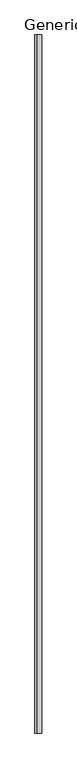
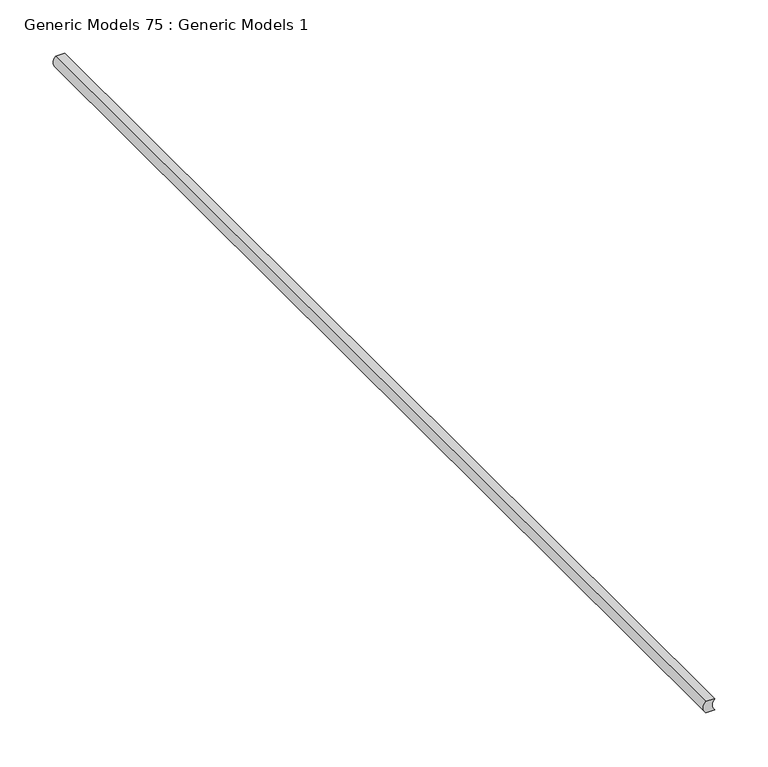
"""IFC4 building model written with IfcOpenShell, lengths in millimetres: proxy geometry, Generic Models 75 : Generic Models 1."""

from ifc_helpers import new_model, si_unit, point, frame, frame_2d, origin, place, context, project, spatial, polyline, circle_curve, trimmed, segment, composite_curve, outline, extrude, source, transform, mapped, element, save


def generic_models_75_generic_models_1_c604be2e(model_context):
    return source(origin(), model_context, "Body", "SweptSolid", [
        extrude(outline(composite_curve([segment(trimmed(circle_curve(frame_2d((2472.600412, 51037.604481)), 8.620055), [point((2466.250412, 51031.775))], [point((2478.950412, 51031.775))], True, "CARTESIAN"), True, "CONTINUOUS"), segment(polyline([(2478.950412, 51031.775), (2478.950412, 51022.25)]), True, "CONTINUOUS"), segment(trimmed(circle_curve(frame_2d((2472.600412, 51028.079481)), 8.620055), [point((2478.950412, 51022.25))], [point((2466.250412, 51022.25))], False, "CARTESIAN"), True, "CONTINUOUS"), segment(polyline([(2466.250412, 51022.25), (2466.250412, 51031.775)]), True, "CONTINUOUS")], self_intersect=False)), frame((0.0, 0.0, 0.0), z_axis=(0.0, 1.0, 0.0), x_axis=(0.0, 0.0, 1.0)), (0.0, 0.0, 1.0), 1219.2),
    ])


if __name__ == "__main__":
    model = new_model("IFC4")
    model_context = context("Model", 3, world=origin())
    ifc_project = project(units=[si_unit("LENGTHUNIT", "METRE", prefix="MILLI")], contexts=[model_context])
    site = spatial("IfcSite", under=ifc_project)
    building = spatial("IfcBuilding", under=site)
    placement = place(None, origin())
    generic_models_75_generic_models_1_shape = generic_models_75_generic_models_1_c604be2e(model_context)
    element("IfcBuildingElementProxy", 1, Name="Generic Models 75 : Generic Models 1", ObjectType="Generic Models 75 : Generic Models 1", at=placement, inside=building, context=model_context, shape_type="MappedRepresentation", body=[
        mapped(generic_models_75_generic_models_1_shape, transform((0.0, 0.0, 0.0), x_axis=(1.0, 0.0, 0.0), y_axis=(0.0, 1.0, 0.0), z_axis=(0.0, 0.0, 1.0))),
    ])
    save(model, "model.ifc")

# Revit data of these elements
# Element 1 (IfcBuildingElementProxy, "Generic Models 75 : Generic Models 1")
#   Materials on its faces: "ACOUSTICAL SEALANT"
# Materials
#   "ACOUSTICAL SEALANT": class "Unassigned", colour RGB 120 120 120, transparency 0, Cost = 0
